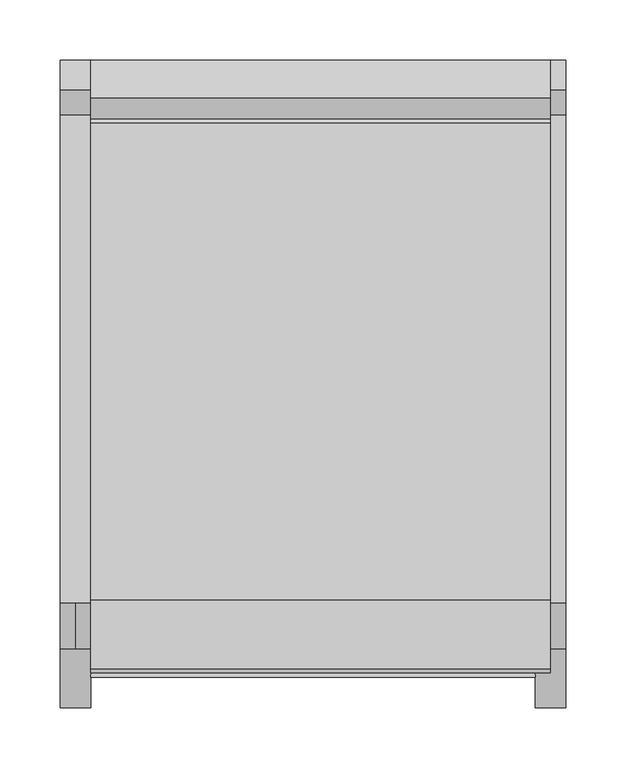
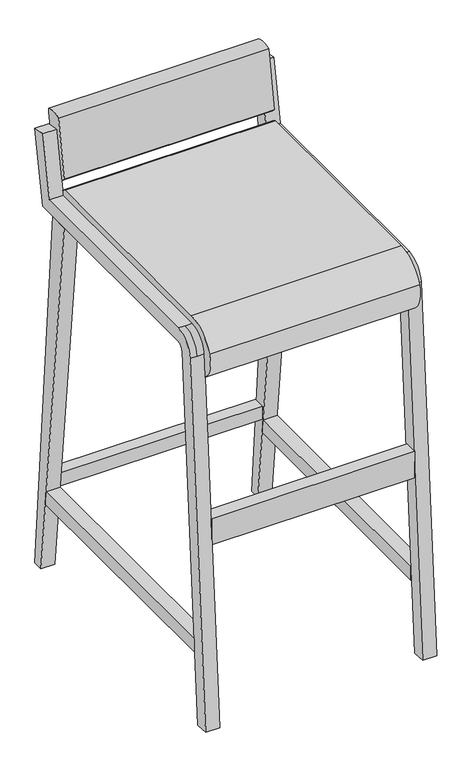
"""IFC4 building model written with IfcOpenShell, lengths in millimetres: furniture geometry, Bar_Stool_6722[1] : Bar_Stool_6722[1]."""

from ifc_helpers import new_model, si_unit, point, frame, frame_2d, origin, place, context, project, spatial, polyline, circle_curve, trimmed, segment, composite_curve, outline, extrude, source, transform, mapped, element, save
from ifc_brep_helpers import plane_surface, cylinder_surface, revolved_surface, advanced_brep


def furniture_9d95edac(model_context):
    return source(origin(), model_context, "Body", "SolidModel", [
        advanced_brep(
        [(419.1, -25.0141169, 838.4759165), (419.1, 0.0, 834.0652528), (393.7, 0.0, 834.0652528), (393.7, -25.0141169, 838.4759165), (393.7, -45.2169423, 723.9), (419.1, -45.2169423, 723.9), (393.7, -23.9038117, 698.5), (393.7, -450.0350637, 698.5), (393.7, -462.7032819, 686.6979128), (393.7, -511.439502, -0.8979128), (393.7, -536.7759384, 0.8979128), (393.7, -488.0397183, 688.4937383), (393.7, -450.0350637, 723.9), (419.1, -23.9038117, 698.5), (419.1, -450.0350637, 723.9), (419.1, -488.0397183, 688.4937383), (419.1, -536.7759384, 0.8979128), (419.1, -511.439502, -0.8979128), (419.1, -462.7032819, 686.6979128), (419.1, -450.0350637, 698.5), (406.4, -450.0350637, 723.9), (406.4, -488.0397183, 688.4937383)],
        [
            (0, 1),
            (1, 2),
            (2, 3),
            (3, 0),
            (3, 4),
            (4, 5),
            (5, 0),
            (2, 6),
            (6, 7),
            (7, 8, circle_curve(frame((393.7, -450.0350637, 685.8), z_axis=(1.0, 0.0, 0.0), x_axis=(0.0, 0.0, 1.0)), 12.7)),
            (8, 9),
            (9, 10),
            (10, 11),
            (11, 12, circle_curve(frame((393.7, -450.0350637, 685.8), z_axis=(-1.0, 0.0, 0.0), x_axis=(0.0, 0.0, 1.0)), 38.1)),
            (12, 4),
            (1, 13),
            (13, 6),
            (5, 14),
            (14, 15, circle_curve(frame((419.1, -450.0350637, 685.8), z_axis=(1.0, 0.0, 0.0), x_axis=(0.0, 0.0, 1.0)), 38.1)),
            (15, 16),
            (16, 17),
            (17, 18),
            (18, 19, circle_curve(frame((419.1, -450.0350637, 685.8), z_axis=(-1.0, 0.0, 0.0), x_axis=(0.0, 0.0, 1.0)), 12.7)),
            (19, 13),
            (12, 20),
            (20, 14),
            (19, 7),
            (21, 15),
            (20, 21, circle_curve(frame((406.4, -450.0350637, 685.8), z_axis=(1.0, 0.0, 0.0), x_axis=(0.0, 0.0, 1.0)), 38.1)),
            (11, 21),
            (18, 8),
            (10, 16),
            (17, 9),
        ],
        [
            plane_surface(frame((406.4, -12.5070585, 836.2705846), z_axis=(0.0, 0.17364817766692853, 0.9848077530122085), x_axis=(1.0, 0.0, 0.0))),
            plane_surface(frame((406.4, -25.0141169, 838.4759165), z_axis=(0.0, -0.9848077530122085, 0.17364817766692814), x_axis=(0.0, -0.17364817766692814, -0.9848077530122085))),
            plane_surface(frame((393.7, -25.0141169, 838.4759165), z_axis=(-1.0, 0.0, 0.0), x_axis=(0.0, -0.17364817766692808, -0.9848077530122085))),
            plane_surface(frame((393.7, 0.0, 834.0652528), z_axis=(0.0, 0.9848077530122085, -0.17364817766692817), x_axis=(0.0, -0.17364817766692817, -0.9848077530122085))),
            plane_surface(frame((419.1, 0.0, 834.0652528), z_axis=(1.0000000000000002, 0.0, 0.0), x_axis=(0.0, -0.1736481776669284, -0.9848077530122085))),
            plane_surface(frame((406.4, -45.2169423, 723.9), z_axis=(0.0, 0.0, 1.0), x_axis=(0.0, -1.0, 0.0))),
            plane_surface(frame((393.7, -23.9038117, 698.5), z_axis=(0.0, 0.0, -1.0), x_axis=(0.0, -1.0, 0.0))),
            cylinder_surface(frame((406.4, -450.0350637, 685.8), z_axis=(-1.0, 0.0, 0.0), x_axis=(0.0, 0.0, 1.0)), 38.1),
            revolved_surface(polyline([(393.7, -450.0350637, 698.5), (419.1, -450.0350637, 698.5)]), (406.4, -450.0350637, 685.8), (-1.0, 0.0, 0.0)),
            plane_surface(frame((406.4, -488.0397183, 688.4937383), z_axis=(0.0, -0.9974974969901172, 0.07070179275273744), x_axis=(0.0, -0.07070179275273744, -0.9974974969901172))),
            plane_surface(frame((393.7, -462.7032819, 686.6979128), z_axis=(0.0, 0.9974974969901172, -0.07070179275273743), x_axis=(0.0, -0.07070179275273743, -0.9974974969901172))),
            plane_surface(frame((406.4, -524.1077202, 0.0), z_axis=(0.0, -0.07070179275273399, -0.9974974969901175), x_axis=(1.0, 0.0, 0.0))),
        ],
        [
            (0, [[1, 2, 3, 4]]),
            (1, [[-4, 5, 6, 7]]),
            (2, [[8, 9, 10, 11, 12, 13, 14, 15, -5, -3]]),
            (3, [[16, 17, -8, -2]]),
            (4, [[-7, 18, 19, 20, 21, 22, 23, 24, -16, -1]]),
            (5, [[-15, 25, 26, -18, -6]]),
            (6, [[-24, 27, -9, -17]]),
            (7, [[28, -19, -26, 29]]),
            (7, [[30, -29, -25, -14]]),
            (8, [[31, -10, -27, -23]]),
            (9, [[32, -20, -28, -30, -13]]),
            (10, [[33, -11, -31, -22]]),
            (11, [[-12, -33, -21, -32]]),
        ],
    ),
        extrude(outline(composite_curve([segment(polyline([(-48.4096386, 756.5644068), (-31.5225381, 863.1853632)]), True, "CONTINUOUS"), segment(trimmed(circle_curve(frame_2d((-15.7612691, 828.3540875)), 38.2313401), [point((-31.5225381, 863.1853632))], [point((0.0, 863.1853632))], False, "CARTESIAN"), True, "CONTINUOUS"), segment(polyline([(0.0, 863.1853632), (0.0, 856.8353632), (-19.1416957, 748.2774126), (-44.0710693, 752.2258375), (-48.4096386, 756.5644068)]), True, "CONTINUOUS")], self_intersect=False)), frame((25.4, 0.0, 0.0), z_axis=(1.0, 0.0, 0.0), x_axis=(0.0, 1.0, 0.0)), (0.0, 0.0, 1.0), 381.0),
        extrude(outline(composite_curve([segment(polyline([(-51.6744261, 737.5144068), (-43.9498561, 733.0546243), (-46.417441, 704.85), (-452.817441, 704.85), (-460.5585493, 681.23302), (-460.5585493, 643.13302), (-484.2663236, 640.1699505)]), True, "CONTINUOUS"), segment(trimmed(circle_curve(frame_2d((-460.5585493, 681.23302)), 47.4155486), [point((-484.2663236, 640.1699505))], [point((-505.1145904, 697.4500928))], False, "CARTESIAN"), True, "CONTINUOUS"), segment(trimmed(circle_curve(frame_2d((-447.8968201, 676.6245275)), 60.8898793), [point((-505.1145904, 697.4500928))], [point((-447.8968201, 737.5144068))], False, "CARTESIAN"), True, "CONTINUOUS"), segment(polyline([(-447.8968201, 737.5144068), (-51.6744261, 737.5144068)]), True, "CONTINUOUS")], self_intersect=False)), frame((25.4, 0.0, 0.0), z_axis=(1.0, 0.0, 0.0), x_axis=(0.0, 1.0, 0.0)), (0.0, 0.0, 1.0), 381.0),
        extrude(outline(polyline([(393.7, -11.6871233), (393.7, -33.1441574), (25.4, -33.1441574), (25.4, -11.6871233), (393.7, -11.6871233)])), frame((0.0, 0.0, 157.9619127), z_axis=(0.0, 0.0, 1.0), x_axis=(1.0, 0.0, 0.0)), (0.0, 0.0, 1.0), 25.4),
        extrude(outline(polyline([(393.7, -488.2695397), (393.7, -511.439502), (25.4, -511.439502), (25.4, -488.2695397), (393.7, -488.2695397)])), frame((0.0, 0.0, 335.7619127), z_axis=(0.0, 0.0, 1.0), x_axis=(1.0, 0.0, 0.0)), (0.0, 0.0, 1.0), 50.8),
        extrude(outline(polyline([(-500.1796497, 157.9619127), (-35.652466, 157.9619127), (-32.9828185, 132.5619127), (-500.1796497, 132.5619127), (-500.1796497, 157.9619127)])), frame((393.7, 0.0, 0.0), z_axis=(1.0, 0.0, 0.0), x_axis=(0.0, 1.0, 0.0)), (0.0, 0.0, 1.0), 25.4),
        extrude(outline(polyline([(-500.1796497, 157.9619127), (-35.652466, 157.9619127), (-32.9828185, 132.5619127), (-500.1796497, 132.5619127), (-500.1796497, 157.9619127)])), frame((0.0, 0.0, 0.0), z_axis=(1.0, 0.0, 0.0), x_axis=(0.0, 1.0, 0.0)), (0.0, 0.0, 1.0), 25.4),
        extrude(outline(polyline([(0.0, 0.0), (-19.05, 0.0), (-92.4653083, 698.5), (-55.3031462, 698.5), (0.0, 0.0)])), frame((393.7, 0.0, 0.0), z_axis=(1.0, 0.0, 0.0), x_axis=(0.0, 1.0, 0.0)), (0.0, 0.0, 1.0), 25.4),
        advanced_brep(
        [(25.4, -25.0141169, 838.4759165), (25.4, 0.0, 834.0652528), (0.0, 0.0, 834.0652528), (0.0, -25.0141169, 838.4759165), (0.0, -45.2169423, 723.9), (25.4, -45.2169423, 723.9), (0.0, -23.9038117, 698.5), (0.0, -450.0350637, 698.5), (0.0, -462.7032819, 686.6979128), (0.0, -511.439502, -0.8979128), (0.0, -536.7759384, 0.8979128), (0.0, -488.0397183, 688.4937383), (0.0, -450.0350637, 723.9), (25.4, -23.9038117, 698.5), (25.4, -450.0350637, 723.9), (25.4, -488.0397183, 688.4937383), (25.4, -536.7759384, 0.8979128), (25.4, -511.439502, -0.8979128), (25.4, -462.7032819, 686.6979128), (25.4, -450.0350637, 698.5), (12.7, -450.0350637, 723.9), (12.7, -488.0397183, 688.4937383)],
        [
            (0, 1),
            (1, 2),
            (2, 3),
            (3, 0),
            (3, 4),
            (4, 5),
            (5, 0),
            (2, 6),
            (6, 7),
            (7, 8, circle_curve(frame((0.0, -450.0350637, 685.8), z_axis=(1.0, 0.0, 0.0), x_axis=(0.0, 0.0, 1.0)), 12.7)),
            (8, 9),
            (9, 10),
            (10, 11),
            (11, 12, circle_curve(frame((0.0, -450.0350637, 685.8), z_axis=(-1.0, 0.0, 0.0), x_axis=(0.0, 0.0, 1.0)), 38.1)),
            (12, 4),
            (1, 13),
            (13, 6),
            (5, 14),
            (14, 15, circle_curve(frame((25.4, -450.0350637, 685.8), z_axis=(1.0, 0.0, 0.0), x_axis=(0.0, 0.0, 1.0)), 38.1)),
            (15, 16),
            (16, 17),
            (17, 18),
            (18, 19, circle_curve(frame((25.4, -450.0350637, 685.8), z_axis=(-1.0, 0.0, 0.0), x_axis=(0.0, 0.0, 1.0)), 12.7)),
            (19, 13),
            (12, 20),
            (20, 14),
            (19, 7),
            (21, 15),
            (20, 21, circle_curve(frame((12.7, -450.0350637, 685.8), z_axis=(1.0, 0.0, 0.0), x_axis=(0.0, 0.0, 1.0)), 38.1)),
            (11, 21),
            (18, 8),
            (10, 16),
            (17, 9),
        ],
        [
            plane_surface(frame((12.7, -12.5070585, 836.2705846), z_axis=(0.0, 0.17364817766692853, 0.9848077530122085), x_axis=(1.0, 0.0, 0.0))),
            plane_surface(frame((12.7, -25.0141169, 838.4759165), z_axis=(0.0, -0.9848077530122085, 0.173648177666928), x_axis=(0.0, -0.173648177666928, -0.9848077530122085))),
            plane_surface(frame((0.0, -25.0141169, 838.4759165), z_axis=(-1.0, 0.0, 0.0), x_axis=(0.0, -0.17364817766692875, -0.9848077530122084))),
            plane_surface(frame((0.0, 0.0, 834.0652528), z_axis=(0.0, 0.9848077530122084, -0.17364817766692883), x_axis=(0.0, -0.17364817766692883, -0.9848077530122084))),
            plane_surface(frame((25.4, 0.0, 834.0652528), z_axis=(1.0000000000000002, 0.0, 0.0), x_axis=(0.0, -0.1736481776669284, -0.9848077530122085))),
            plane_surface(frame((12.7, -45.2169423, 723.9), z_axis=(0.0, 0.0, 1.0), x_axis=(0.0, -1.0, 0.0))),
            plane_surface(frame((0.0, -23.9038117, 698.5), z_axis=(0.0, 0.0, -1.0), x_axis=(0.0, -1.0, 0.0))),
            cylinder_surface(frame((12.7, -450.0350637, 685.8), z_axis=(-1.0, 0.0, 0.0), x_axis=(0.0, 0.0, 1.0)), 38.1),
            revolved_surface(polyline([(0.0, -450.0350637, 698.5), (25.4, -450.0350637, 698.5)]), (12.7, -450.0350637, 685.8), (-1.0, 0.0, 0.0)),
            plane_surface(frame((12.7, -488.0397183, 688.4937383), z_axis=(0.0, -0.9974974969901172, 0.07070179275273744), x_axis=(0.0, -0.07070179275273744, -0.9974974969901172))),
            plane_surface(frame((0.0, -462.7032819, 686.6979128), z_axis=(0.0, 0.9974974969901172, -0.07070179275273743), x_axis=(0.0, -0.07070179275273743, -0.9974974969901172))),
            plane_surface(frame((12.7, -524.1077202, 0.0), z_axis=(0.0, -0.07070179275273399, -0.9974974969901175), x_axis=(1.0, 0.0, 0.0))),
        ],
        [
            (0, [[1, 2, 3, 4]]),
            (1, [[-4, 5, 6, 7]]),
            (2, [[8, 9, 10, 11, 12, 13, 14, 15, -5, -3]]),
            (3, [[16, 17, -8, -2]]),
            (4, [[-7, 18, 19, 20, 21, 22, 23, 24, -16, -1]]),
            (5, [[-15, 25, 26, -18, -6]]),
            (6, [[-24, 27, -9, -17]]),
            (7, [[28, -19, -26, 29]]),
            (7, [[30, -29, -25, -14]]),
            (8, [[31, -10, -27, -23]]),
            (9, [[32, -20, -28, -30, -13]]),
            (10, [[33, -11, -31, -22]]),
            (11, [[-12, -33, -21, -32]]),
        ],
    ),
        extrude(outline(polyline([(0.0, 0.0), (-19.05, 0.0), (-92.4653083, 698.5), (-55.3031462, 698.5), (0.0, 0.0)])), frame((0.0, 0.0, 0.0), z_axis=(1.0, 0.0, 0.0), x_axis=(0.0, 1.0, 0.0)), (0.0, 0.0, 1.0), 25.4),
    ])


if __name__ == "__main__":
    model = new_model("IFC4")
    model_context = context("Model", 3, world=origin())
    ifc_project = project(units=[si_unit("LENGTHUNIT", "METRE", prefix="MILLI")], contexts=[model_context])
    site = spatial("IfcSite", under=ifc_project)
    building = spatial("IfcBuilding", under=site)
    placement = place(None, origin())
    furniture_shape = furniture_9d95edac(model_context)
    element("IfcFurniture", 1, ObjectType="Bar_Stool_6722[1] : Bar_Stool_6722[1]", at=placement, inside=building, context=model_context, shape_type="MappedRepresentation", body=[
        mapped(furniture_shape, transform((0.0, 0.0, 0.0), x_axis=(1.0, 0.0, 0.0), y_axis=(0.0, 1.0, 0.0), z_axis=(0.0, 0.0, 1.0))),
    ])
    save(model, "model.ifc")

# Revit data of these elements
# Type "Bar_Stool_6722[1] : Bar_Stool_6722[1]"
#   Seat = fab
#   Chair Legs = MET
# Element 1 (IfcFurniture, "Bar_Stool_6722[1] : Bar_Stool_6722[1]")
#   Materials on its faces: "MET", "fab"
# Materials
#   "fab": class "Leather", colour RGB 255 255 255, transparency 0, Cost = 0
#   "MET": class "Metal", colour RGB 189 187 185, transparency 0
